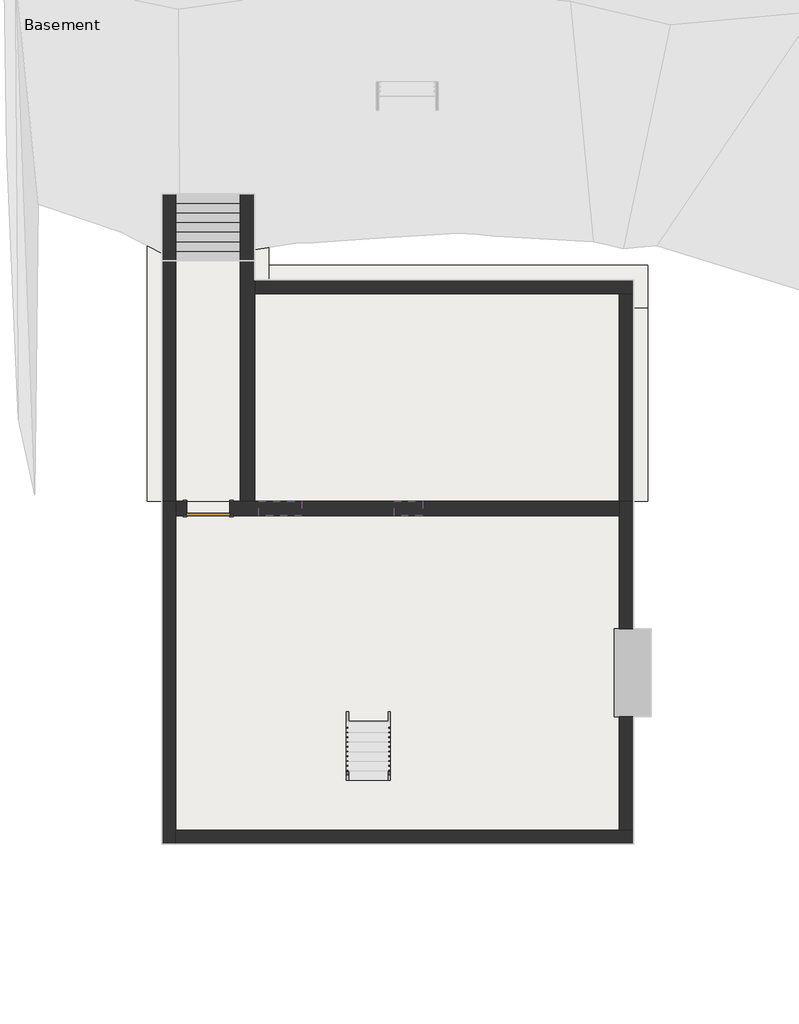
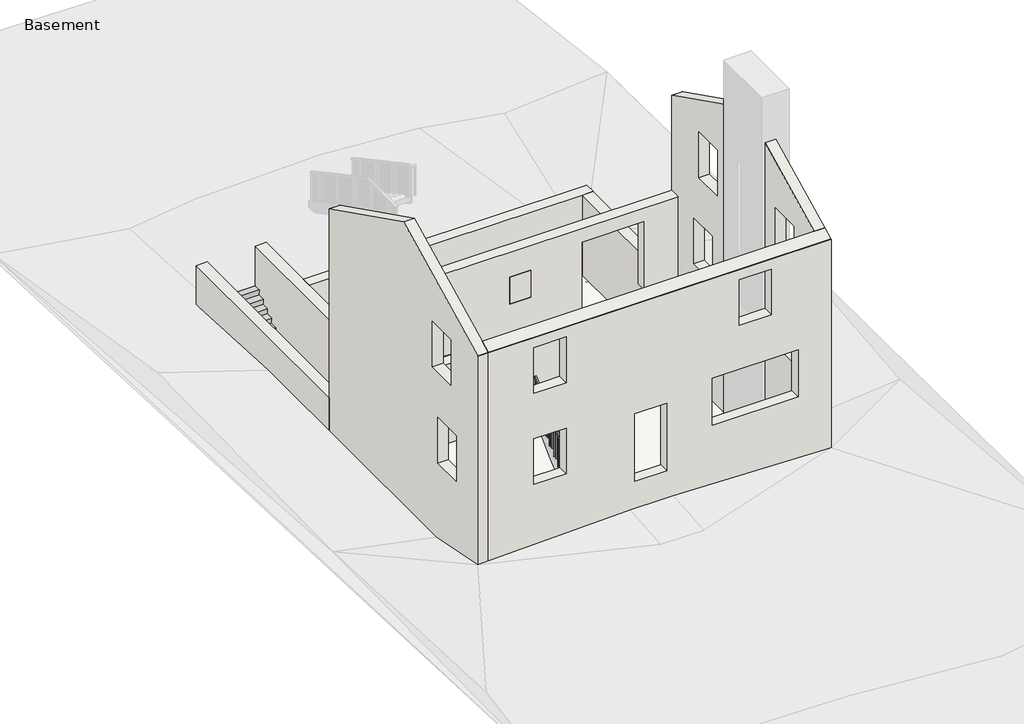
# One storey, part 1 of 2: 11 walls, 4 footings, 4 slabs, 2 railings, 1 door, 1 stair flight.
# Revit data of these elements (continued)
# Elements 6, 7 (IfcRailing, "Handrail - Rectangular") (continued)
#   Phase Created = Existing
# Element 8 (IfcSlab, "4\" Concrete")
#   built-in parameter 1001955 = 1.5708 (stored number, unit not read)
#   Height Offset From Level = 0' - 0"
#   Phase Created = New Construction
#   Materials on its faces: "Concrete, Lightweight"
# Elements 9, 10 (IfcSlab, "Pad 1")
#   built-in parameter 1012502 = -0.333333 (stored number, unit not read)
#   Phase Created = New Construction
# Element 11 (IfcSlab, "Pad 1")
#   built-in parameter 1012502 = -1.33333 (stored number, unit not read)
#   Phase Created = New Construction
# Element 12 (IfcStairFlight, "3/4\" Nosing")
#   Phase Created = New Construction
#   Materials on its faces: "Concrete, Cast-in-Place gray"
# Elements 13, 14, 15, 16 (IfcWall, "Foundation - 12\" Concrete")
#   built-in parameter 1001111 = -0' - 4"
#   Top Offset = 0' - 0"
#   Base Offset = -0' - 4"
#   wall height = 7' - 11 1/4"
#   Phase Created = New Construction
#   Base Constraint = Basement
#   Top Constraint = Top of Foundation
#   Materials on its faces: "Concrete, Cast-in-Place gray"
# Element 17 (IfcWall, "Generic - 12\"")
#   Top Offset = 0' - 0"
#   Base Offset = 0' - 0"
#   wall height = 17' - 9"
#   Phase Created = Existing
#   Base Constraint = Basement
#   Top Constraint = Second Floor
#   Materials on its faces: "Default Wall"
# Elements 18, 19, 20, 21 (IfcWall, "Generic - 12\"")
#   Top Offset = 0' - 0"
#   Base Offset = 0' - 0"
#   wall height = 26' - 9"
#   Phase Created = Existing
#   Base Constraint = Basement
#   Top Constraint = Roof
#   Materials on its faces: "Default Wall"
# Elements 22, 23 (IfcWall, "Generic - 12\"")
#   Top Offset = 0' - 0"
#   Base Offset = 0' - 0"
#   Unconnected Height = 17' - 9"
#   wall height = 17' - 9"
#   Phase Created = New Construction
#   Base Constraint = Basement
#   Top Constraint = Basement
#   Materials on its faces: "Default Wall"
# Materials
#   "Door - Panel": class "Wood", colour RGB 210 159 95, transparency 0, Cost = 0
#   "Door - Frame": class "Miscellaneous", colour RGB 118 70 51, transparency 0, Cost = 0
#   "Concrete, Lightweight": class "Concrete", colour RGB 142 141 140, transparency 0, Description = "Lightweight concrete", Cost = 0
#   "Concrete, Cast-in-Place gray": class "Concrete", colour RGB 192 192 192, transparency 0, Description = "Cast-in-place concrete", Cost = 0
#   "Default Wall": class "Miscellaneous", colour RGB 128 128 128, transparency 0, Cost = 0
